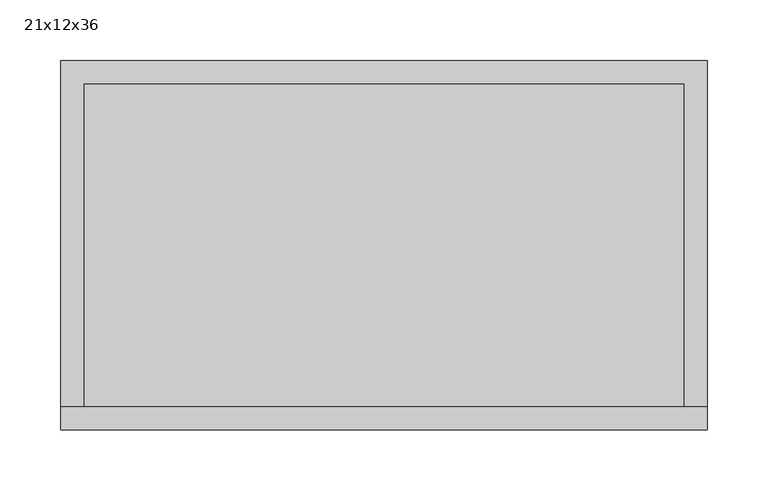
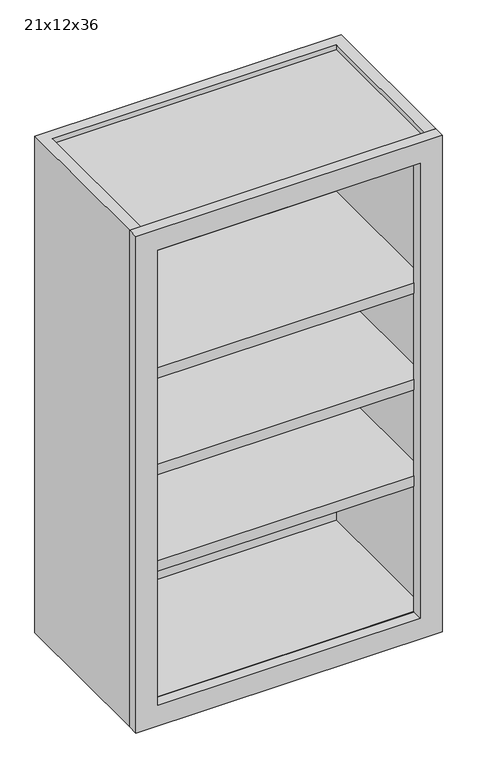
"""IFC4 building model written with IfcOpenShell, lengths in millimetres: furniture geometry, Bookcase-Merillat : 21x12x36."""

from ifc_helpers import new_model, si_unit, frame, origin, place, context, project, spatial, polyline, outline, extrude, faceted_brep, source, transform, mapped, element, save


def furniture_21x12x36_620eb8e4(model_context):
    return source(origin(), model_context, "Body", "SolidModel", [
        extrude(outline(polyline([(-247.65, 133.35), (247.65, 133.35), (247.65, -133.35), (-247.65, -133.35), (-247.65, 133.35)])), frame((0.0, 0.0, 269.875), z_axis=(0.0, 0.0, 1.0), x_axis=(1.0, 0.0, 0.0)), (0.0, 0.0, 1.0), 19.3909952),
        extrude(outline(polyline([(-247.65, 133.35), (247.65, 133.35), (247.65, -133.35), (-247.65, -133.35), (-247.65, 133.35)])), frame((0.0, 0.0, 625.1340048), z_axis=(0.0, 0.0, 1.0), x_axis=(1.0, 0.0, 0.0)), (0.0, 0.0, 1.0), 19.3909952),
        extrude(outline(polyline([(-247.65, 133.35), (247.65, 133.35), (247.65, -133.35), (-247.65, -133.35), (-247.65, 133.35)])), frame((0.0, 0.0, 447.5180074), z_axis=(0.0, 0.0, 1.0), x_axis=(1.0, 0.0, 0.0)), (0.0, 0.0, 1.0), 19.3909952),
        extrude(outline(polyline([(-247.65, 133.35), (247.65, 133.35), (247.65, -133.35), (-247.65, -133.35), (-247.65, 133.35)])), frame((0.0, 0.0, 19.3909952), z_axis=(0.0, 0.0, 1.0), x_axis=(1.0, 0.0, 0.0)), (0.0, 0.0, 1.0), 19.3909952),
        extrude(outline(polyline([(0.0, -266.7), (0.0, 266.7), (914.4, 266.7), (914.4, -266.7), (0.0, -266.7)]), holes=[polyline([(876.3, -228.6), (876.3, 228.6), (38.1, 228.6), (38.1, -228.6), (876.3, -228.6)])]), frame((0.0, -152.4, 0.0), z_axis=(0.0, 1.0, 0.0), x_axis=(0.0, 0.0, 1.0)), (0.0, 0.0, 1.0), 19.05),
        faceted_brep([(-247.65, -133.35, 19.3909952), (247.65, -133.35, 19.3909952), (247.65, 133.35, 19.3909952), (-247.65, 133.35, 19.3909952), (-266.7, 152.4, 0.0), (266.7, 152.4, 0.0), (266.7, -133.35, 0.0), (-266.7, -133.35, 0.0), (-266.7, -133.35, 914.4), (266.7, -133.35, 914.4), (247.65, -133.35, 914.4), (247.65, -133.35, 905.1909423), (-247.65, -133.35, 905.1909423), (-247.65, -133.35, 914.4), (-247.65, -133.35, 895.0090048), (247.65, -133.35, 895.0090048), (-247.65, 133.35, 905.1909423), (247.65, 133.35, 905.1909423), (-247.65, 133.35, 914.4), (247.65, 133.35, 914.4), (-266.7, 152.4, 914.4), (266.7, 152.4, 914.4), (-247.65, 133.35, 895.0090048), (247.65, 133.35, 895.0090048)], [[[0, 1, 2, 3]], [[4, 5, 6, 7]], [[8, 7, 6, 9, 10, 11, 12, 13], [1, 0, 14, 15]], [[16, 12, 11, 17]], [[12, 16, 18, 13]], [[17, 11, 10, 19]], [[16, 17, 19, 18]], [[20, 8, 13, 18, 19, 10, 9, 21]], [[8, 20, 4, 7]], [[0, 3, 22, 14]], [[3, 2, 23, 22]], [[2, 1, 15, 23]], [[21, 9, 6, 5]], [[20, 21, 5, 4]], [[15, 14, 22, 23]]]),
    ])


if __name__ == "__main__":
    model = new_model("IFC4")
    model_context = context("Model", 3, world=origin())
    ifc_project = project(units=[si_unit("LENGTHUNIT", "METRE", prefix="MILLI")], contexts=[model_context])
    site = spatial("IfcSite", under=ifc_project)
    building = spatial("IfcBuilding", under=site)
    placement = place(None, origin())
    furniture_21x12x36_shape = furniture_21x12x36_620eb8e4(model_context)
    element("IfcFurniture", 1, ObjectType="Bookcase-Merillat : 21x12x36", at=placement, inside=building, context=model_context, shape_type="MappedRepresentation", body=[
        mapped(furniture_21x12x36_shape, transform((0.0, 0.0, 0.0), x_axis=(1.0, 0.0, 0.0), y_axis=(0.0, 1.0, 0.0), z_axis=(0.0, 0.0, 1.0))),
    ])
    save(model, "model.ifc")

# Revit data of these elements
# Type "Bookcase-Merillat : 21x12x36"
#   URL = "https://www.merillat.com/"
#   Product Page URL = "https://www.merillat.com/our-products/"
#   Product Documentation Link = "http://merillatbusiness.com/wp-content/uploads/2014/07/Merillat_Classic_Catalog.pdf"
#   Model = "BK2136"
#   Manufacturer = "Merillat"
#   Description = "Bookcase"
#   Construction Type = "Bookcase"
#   Assembly Code = "E2020200"
#   Width = 1' - 9"
#   Shelving Height = 0' - 11"
#   Height = 3' - 0"
#   Depth = 1' - 0"
#   Default Elevation = 4' - 0"
#   Cabinet Shell = 0' - 0 3/4"
#   COBie.Type = no
#   Two Drawer = yes
#   Shelves Bookcase = yes
#   Number of Shelves = 2
#   No Shelf Bookcase = no
#   Middle Shelf = yes
#   Shelving Material = Wood - Merillat - Pecan(1)
#   Bookcase Material = Wood - Merillat - Pecan(1)
# Element 1 (IfcFurniture, "Bookcase-Merillat : 21x12x36")
#   Materials on its faces: "Wood - Merillat - Pecan(1)"
# Materials
#   "Wood - Merillat - Pecan(1)": class "Wood", colour RGB 108 67 43, transparency 0, Cost = 0
